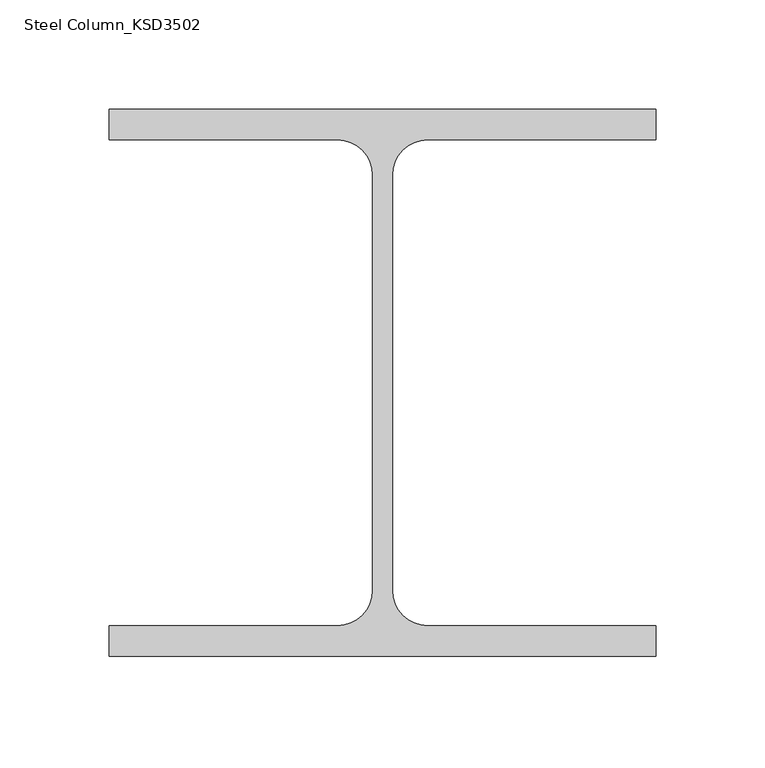
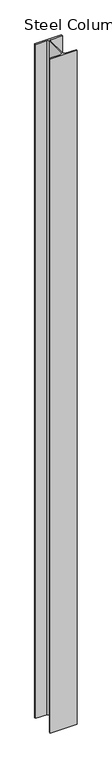
"""IFC4 building model written with IfcOpenShell, lengths in millimetres: column geometry, Steel Column_KSD3502 : H_SC_ASC_H-250×250x9x14."""

from ifc_helpers import new_model, si_unit, point, frame, frame_2d, origin, place, context, project, spatial, polyline, circle_curve, trimmed, segment, composite_curve, outline, extrude, source, transform, mapped, element, save


def steel_column_ksd3502_8fa00422(model_context):
    return source(origin(), model_context, "Body", "SweptSolid", [
        extrude(outline(composite_curve([segment(polyline([(125.0, 125.0), (125.0, 111.0), (20.5, 111.0)]), True, "CONTINUOUS"), segment(trimmed(circle_curve(frame_2d((20.5, 95.0)), 16.0), [point((20.5, 111.0))], [point((4.5, 95.0))], True, "CARTESIAN"), True, "CONTINUOUS"), segment(polyline([(4.5, 95.0), (4.5, -95.0)]), True, "CONTINUOUS"), segment(trimmed(circle_curve(frame_2d((20.5, -95.0)), 16.0), [point((4.5, -95.0))], [point((20.5, -111.0))], True, "CARTESIAN"), True, "CONTINUOUS"), segment(polyline([(20.5, -111.0), (125.0, -111.0), (125.0, -125.0), (-125.0, -125.0), (-125.0, -111.0), (-20.5, -111.0)]), True, "CONTINUOUS"), segment(trimmed(circle_curve(frame_2d((-20.5, -95.0)), 16.0), [point((-20.5, -111.0))], [point((-4.5, -95.0))], True, "CARTESIAN"), True, "CONTINUOUS"), segment(polyline([(-4.5, -95.0), (-4.5, 95.0)]), True, "CONTINUOUS"), segment(trimmed(circle_curve(frame_2d((-20.5, 95.0)), 16.0), [point((-4.5, 95.0))], [point((-20.5, 111.0))], True, "CARTESIAN"), True, "CONTINUOUS"), segment(polyline([(-20.5, 111.0), (-125.0, 111.0), (-125.0, 125.0), (125.0, 125.0)]), True, "CONTINUOUS")], self_intersect=False)), frame((0.0, 0.0, 599.9720055), z_axis=(0.0, 0.0, 1.0), x_axis=(1.0, 0.0, 0.0)), (0.0, 0.0, 1.0), 6600.0),
    ])


if __name__ == "__main__":
    model = new_model("IFC4")
    model_context = context("Model", 3, world=origin())
    ifc_project = project(units=[si_unit("LENGTHUNIT", "METRE", prefix="MILLI")], contexts=[model_context])
    site = spatial("IfcSite", under=ifc_project)
    building = spatial("IfcBuilding", under=site)
    placement = place(None, origin())
    steel_column_ksd3502_shape = steel_column_ksd3502_8fa00422(model_context)
    element("IfcColumn", 1, ObjectType="Steel Column_KSD3502 : H_SC_ASC_H-250×250x9x14", at=placement, inside=building, context=model_context, shape_type="MappedRepresentation", body=[
        mapped(steel_column_ksd3502_shape, transform((0.0, 0.0, 0.0), x_axis=(1.0, 0.0, 0.0), y_axis=(0.0, 1.0, 0.0), z_axis=(0.0, 0.0, 1.0))),
    ])
    save(model, "model.ifc")

# Revit data of these elements
# Type "Steel Column_KSD3502 : H_SC_ASC_H-250×250x9x14"
#   Width = 25.0 cm
#   Web Thickness = 0.9 cm
#   Web Fillet = 1.6 cm
#   Warping Constant = 507646.0 cm⁶
#   Torsional Moment of Inertia = 51.4681 cm⁴
#   Section Area = 92.18 cm²
#   Plastic Modulus weak axis = 444.0 cm³
#   Plastic Modulus strong axis = 960.0 cm³
#   Perimeter = 1.27 m²/m
#   Nominal Weight = 72.40 kgf/m
#   Moment of Inertia weak axis = 3650.00 cm⁴
#   Moment of Inertia strong axis = 10800.00 cm⁴
#   Height = 25.0 cm
#   Flange Thickness = 1.4 cm
#   Elastic Modulus weak axis = 292.0 cm³
#   Elastic Modulus strong axis = 867.0 cm³
#   Centroid Vertical = 12.5 cm
#   Centroid Horizontal = 12.5 cm
#   Bolt Spacing = 13.97 cm
#   Structural Material [instance default] = Steel, 45-345
#   Section Name Key = ""
#   Assembly Code = ""
# Element 1 (IfcColumn, "Steel Column_KSD3502 : H_SC_ASC_H-250×250x9x14")
#   Structural Material = A03AD029-00005_Anchor Bolt (Installation only)_M24
#   Materials on its faces: "A03AD029-00005_Anchor Bolt (Installation only)_M24"
# Materials
#   "Steel, 45-345": class "Metal", colour RGB 189 187 185, transparency 0, Description = "Steel 345 MPa", Cost = 0
#   "A03AD029-00005_Anchor Bolt (Installation only)_M24": class "Unassigned", colour RGB 84 83 81, transparency 0, Cost = 0
